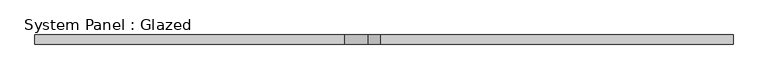
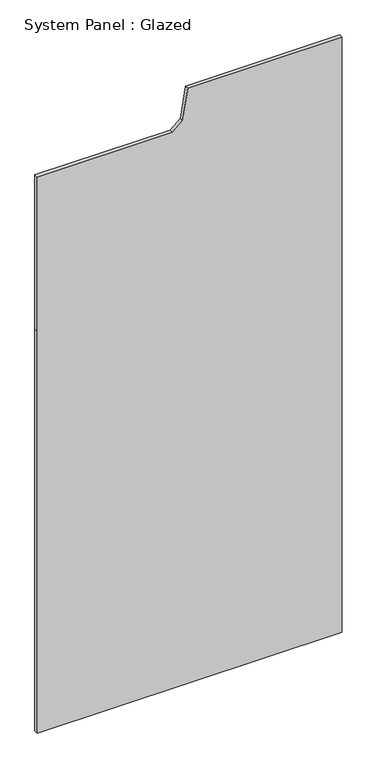
"""IFC4 building model written with IfcOpenShell, lengths in millimetres: plate geometry, System Panel : Glazed."""

from ifc_helpers import new_model, si_unit, frame, origin, place, context, project, spatial, polyline, outline, extrude, source, transform, mapped, element, save


def system_panel_glazed_1e4dd7ae(model_context):
    return source(origin(), model_context, "Body", "SweptSolid", [
        extrude(outline(polyline([(0.0, -739.9886538), (0.0, 739.9886538), (2060.0, 739.9886538), (3050.0, 739.9886538), (3050.0, -8.3597927), (2892.1782767, -33.356298), (2850.0, -82.7407151), (2850.0, -739.9886538), (2060.0, -739.9886538), (0.0, -739.9886538)])), frame((0.0, 0.0, 0.0), z_axis=(0.0, 1.0, 0.0), x_axis=(0.0, 0.0, 1.0)), (0.0, 0.0, 1.0), 20.0),
    ])


if __name__ == "__main__":
    model = new_model("IFC4")
    model_context = context("Model", 3, world=origin())
    ifc_project = project(units=[si_unit("LENGTHUNIT", "METRE", prefix="MILLI")], contexts=[model_context])
    site = spatial("IfcSite", under=ifc_project)
    building = spatial("IfcBuilding", under=site)
    placement = place(None, origin())
    system_panel_glazed_shape = system_panel_glazed_1e4dd7ae(model_context)
    element("IfcPlate", 1, ObjectType="System Panel : Glazed", at=placement, inside=building, context=model_context, shape_type="MappedRepresentation", body=[
        mapped(system_panel_glazed_shape, transform((0.0, 0.0, 0.0), x_axis=(1.0, 0.0, 0.0), y_axis=(0.0, 1.0, 0.0), z_axis=(0.0, 0.0, 1.0))),
    ])
    save(model, "model.ifc")

# Revit data of these elements
# Type "System Panel : Glazed"
#   COBie.Type = no
# Element 1 (IfcPlate, "System Panel : Glazed")
#   Materials on its faces: "Glass"
# Materials
#   "Glass": class "Glass", colour RGB 0 128 192, transparency 0.75, Description = "Soda Lime Glass", Cost = 0
